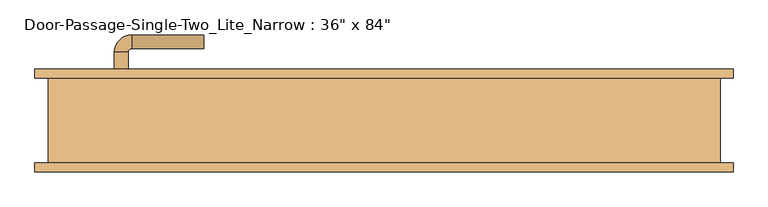
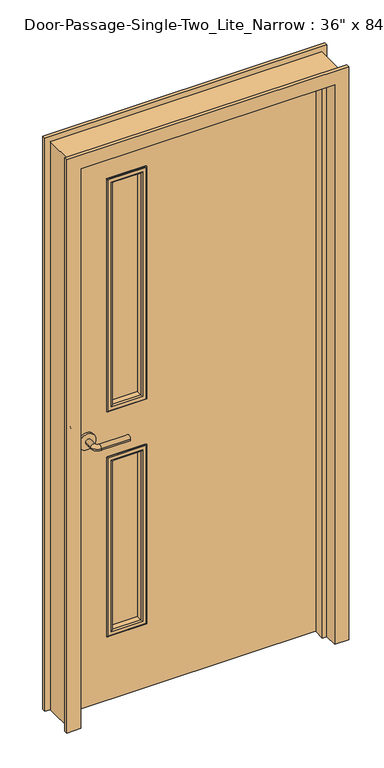
"""IFC4 building model written with IfcOpenShell, lengths in millimetres: door geometry."""

import ifcopenshell
import ifcopenshell.guid

model = None  # the IFC model being written
_history = None  # IfcOwnerHistory: only IFC2X3 demands one
_inside = {}  # id of a spatial element -> (the spatial element, [elements in it])
_under = {}  # id of a project, library or spatial element -> (it, [spatial elements below it])
_declared = {}  # id of a project -> (the project, [libraries it declares])
_typed = {}  # id of a type object -> (the type object, [elements of that type])
_made_of = {}  # id of a material, layer set ... -> (it, [elements and type objects made of it])


def new_model(schema):
    """Start an empty IFC model of exactly this schema.

    Asked for "IFC4X3", IfcOpenShell would pick the latest addendum, in which some entities
    have other attributes; the version numbers below select the first issue.
    IFC2X3 requires an IfcOwnerHistory on every rooted entity: one is made here for all.
    """
    global model, _history
    if schema == "IFC4X3":
        model = ifcopenshell.file(schema_version=(4, 3, 0, 0))
    else:
        model = ifcopenshell.file(schema=schema)
    _inside.clear()
    _under.clear()
    _declared.clear()
    _typed.clear()
    _made_of.clear()
    _history = None
    if model.schema == "IFC2X3":
        org = make("IfcOrganization", Name="unknown")
        user = make(
            "IfcPersonAndOrganization",
            ThePerson=make("IfcPerson", FamilyName="unknown"),
            TheOrganization=org,
        )
        app = make(
            "IfcApplication",
            ApplicationDeveloper=org,
            Version="unknown",
            ApplicationFullName="unknown",
            ApplicationIdentifier="unknown",
        )
        _history = make(
            "IfcOwnerHistory",
            OwningUser=user,
            OwningApplication=app,
            ChangeAction="ADDED",
            CreationDate=0,
        )
    return model


def make(cls, **values):
    """One entity of the class cls with the attributes given. An attribute that is None is left unset."""
    return model.create_entity(
        cls, **{name: value for name, value in values.items() if value is not None}
    )


def rooted(cls, **values):
    """An entity with a GlobalId (a new one), such as an element, a storey or a relation."""
    return make(cls, GlobalId=ifcopenshell.guid.new(), OwnerHistory=_history, **values)


def si_unit(unit_type, name, prefix=None):
    """IfcSIUnit, for example si_unit("LENGTHUNIT", "METRE", prefix="MILLI")."""
    return make("IfcSIUnit", UnitType=unit_type, Prefix=prefix, Name=name)


def assignment(units):
    """IfcUnitAssignment: the units of a project."""
    return None if units is None else make("IfcUnitAssignment", Units=units)


def point(xyz):
    """IfcCartesianPoint."""
    return None if xyz is None else make("IfcCartesianPoint", Coordinates=xyz)


def direction(xyz):
    """IfcDirection."""
    return None if xyz is None else make("IfcDirection", DirectionRatios=xyz)


def frame(location, z_axis=None, x_axis=None):
    """IfcAxis2Placement3D, a coordinate frame: its origin and axes. An axis left out is left unset."""
    return make(
        "IfcAxis2Placement3D",
        Location=point(location),
        Axis=direction(z_axis),
        RefDirection=direction(x_axis),
    )


def frame_2d(location, x_axis=None):
    """IfcAxis2Placement2D, a coordinate frame in the plane: its origin and x axis."""
    return make(
        "IfcAxis2Placement2D", Location=point(location), RefDirection=direction(x_axis)
    )


def origin():
    """The frame at (0, 0, 0) with its axes left unset."""
    return frame((0.0, 0.0, 0.0))


def place(relative_to, where):
    """IfcLocalPlacement: puts the frame where relative to a parent placement (None: the world)."""
    return make(
        "IfcLocalPlacement", PlacementRelTo=relative_to, RelativePlacement=where
    )


def context(
    kind, dimensions, precision=None, world=None, true_north=None, identifier=None
):
    """IfcGeometricRepresentationContext, for example the 3D "Model" context."""
    return make(
        "IfcGeometricRepresentationContext",
        ContextIdentifier=identifier,
        ContextType=kind,
        CoordinateSpaceDimension=dimensions,
        Precision=precision,
        WorldCoordinateSystem=world,
        TrueNorth=true_north,
    )


def project(units=None, contexts=None):
    """IfcProject with its units and contexts."""
    return rooted(
        "IfcProject",
        Name="project",
        RepresentationContexts=contexts,
        UnitsInContext=assignment(units),
    )


def spatial(cls, under=None, at=None, **own):
    """A site, building, storey or space (cls), placed at a placement, below another one or the project."""
    s = rooted(cls, ObjectPlacement=at, **own)
    if under is not None:
        _under.setdefault(under.id(), (under, []))[1].append(s)
    return s


def polyline(points):
    """IfcPolyline through the points."""
    return make("IfcPolyline", Points=[point(p) for p in points])


def circle_curve(where, radius):
    """IfcCircle in the frame where."""
    return make("IfcCircle", Position=where, Radius=radius)


def ellipse_curve(where, semi_axis1, semi_axis2):
    """IfcEllipse in the frame where."""
    return make(
        "IfcEllipse", Position=where, SemiAxis1=semi_axis1, SemiAxis2=semi_axis2
    )


def trimmed(basis, trim1, trim2, sense, master):
    """IfcTrimmedCurve: the piece of a basis curve between two trims."""
    return make(
        "IfcTrimmedCurve",
        BasisCurve=basis,
        Trim1=trim1,
        Trim2=trim2,
        SenseAgreement=sense,
        MasterRepresentation=master,
    )


def segment(curve, same_sense, transition):
    """IfcCompositeCurveSegment."""
    return make(
        "IfcCompositeCurveSegment",
        Transition=transition,
        SameSense=same_sense,
        ParentCurve=curve,
    )


def composite_curve(segments, self_intersect=None):
    """IfcCompositeCurve: segments joined end to end."""
    return make("IfcCompositeCurve", Segments=segments, SelfIntersect=self_intersect)


def outline(outer, holes=None, kind="AREA"):
    """IfcArbitraryClosedProfileDef: a profile drawn as a closed curve; with holes, ...WithVoids."""
    if holes is None:
        return make("IfcArbitraryClosedProfileDef", ProfileType=kind, OuterCurve=outer)
    return make(
        "IfcArbitraryProfileDefWithVoids",
        ProfileType=kind,
        OuterCurve=outer,
        InnerCurves=holes,
    )


def extrude(swept, where, along, depth):
    """IfcExtrudedAreaSolid: the profile swept, set in the frame where, extruded along a direction by depth."""
    return make(
        "IfcExtrudedAreaSolid",
        SweptArea=swept,
        Position=where,
        ExtrudedDirection=direction(along),
        Depth=depth,
    )


def faces_of(points, faces, orient=None, outer=None):
    """IfcFace entities. A face is a list of loops; a loop is a list of indices into points, from 0.

    orient and outer hold one flag for each loop. By default every Orientation is true, the
    first loop of a face is its IfcFaceOuterBound and the others are IfcFaceBound.
    """
    made = []
    for i, loops in enumerate(faces):
        bounds = []
        for j, loop in enumerate(loops):
            is_outer = j == 0 if outer is None else outer[i][j]
            bounds.append(
                make(
                    "IfcFaceOuterBound" if is_outer else "IfcFaceBound",
                    Bound=make("IfcPolyLoop", Polygon=[points[k] for k in loop]),
                    Orientation=True if orient is None else orient[i][j],
                )
            )
        made.append(make("IfcFace", Bounds=bounds))
    return made


def faceted_brep(points, faces, orient=None, outer=None, voids=None):
    """IfcFacetedBrep: a solid bounded by flat faces; with voids (closed shells), ...WithVoids."""
    shared = [point(p) for p in points]
    hull = make("IfcClosedShell", CfsFaces=faces_of(shared, faces, orient, outer))
    if voids is None:
        return make("IfcFacetedBrep", Outer=hull)
    return make(
        "IfcFacetedBrepWithVoids",
        Outer=hull,
        Voids=[
            make(cls, CfsFaces=faces_of(shared, fs, o, b)) for cls, fs, o, b in voids
        ],
    )


def shape(context_of_items, identifier, shape_type, items):
    """IfcShapeRepresentation: the items that make up one representation, for example the "Body"."""
    return make(
        "IfcShapeRepresentation",
        ContextOfItems=context_of_items,
        RepresentationIdentifier=identifier,
        RepresentationType=shape_type,
        Items=items,
    )


def source(mapping_origin, context_of_items, identifier, shape_type, items):
    """IfcRepresentationMap: a shape defined once, which mapped items show again and again."""
    return make(
        "IfcRepresentationMap",
        MappingOrigin=mapping_origin,
        MappedRepresentation=shape(context_of_items, identifier, shape_type, items),
    )


def transform(
    local_origin,
    x_axis=None,
    y_axis=None,
    z_axis=None,
    scale=None,
    scale2=None,
    scale3=None,
    uniform=True,
):
    """IfcCartesianTransformationOperator3D, or its non-uniform kind. x_axis, y_axis, z_axis: its Axis1, 2, 3."""
    if uniform:
        return make(
            "IfcCartesianTransformationOperator3D",
            Axis1=direction(x_axis),
            Axis2=direction(y_axis),
            LocalOrigin=point(local_origin),
            Scale=scale,
            Axis3=direction(z_axis),
        )
    return make(
        "IfcCartesianTransformationOperator3DnonUniform",
        Axis1=direction(x_axis),
        Axis2=direction(y_axis),
        LocalOrigin=point(local_origin),
        Scale=scale,
        Axis3=direction(z_axis),
        Scale2=scale2,
        Scale3=scale3,
    )


def mapped(mapping_source, mapping_target):
    """IfcMappedItem: shows the shape of a source again, moved by a transform."""
    return make(
        "IfcMappedItem", MappingSource=mapping_source, MappingTarget=mapping_target
    )


def made_of(thing, what):
    """Note that an element or type object is made of a material, layer set ...; save() writes the relation."""
    if what is not None:
        _made_of.setdefault(what.id(), (what, []))[1].append(thing)
    return thing


def element(
    cls,
    number,
    at=None,
    inside=None,
    cuts=None,
    type_object=None,
    material=None,
    context=None,
    identifier="Body",
    shape_type=None,
    held_by="IfcProductDefinitionShape",
    body=None,
    shapes=None,
    **own,
):
    """One element of the class cls, such as IfcWall. Its Tag is "e" and its number.

    at: its placement. inside: the storey or other place that contains it. cuts: it is an
    opening in that element (IfcRelVoidsElement). A single representation is given by context,
    identifier, shape_type and body (its items); several are given by shapes. held_by: the class
    of the entity that holds the representations. save() writes the other relations.
    """
    e = rooted(cls, Tag="e%d" % number, ObjectPlacement=at, **own)
    if body is not None:
        shapes = [shape(context, identifier, shape_type, body)]
    if shapes is not None:
        e.Representation = make(held_by, Representations=shapes)
    if inside is not None:
        _inside.setdefault(inside.id(), (inside, []))[1].append(e)
    if cuts is not None:
        rooted(
            "IfcRelVoidsElement", RelatingBuildingElement=cuts, RelatedOpeningElement=e
        )
    if type_object is not None:
        _typed.setdefault(type_object.id(), (type_object, []))[1].append(e)
    return made_of(e, material)


def aggregate(whole, parts):
    """IfcRelAggregates: a whole, such as a stair, and the parts it consists of."""
    return rooted("IfcRelAggregates", RelatingObject=whole, RelatedObjects=parts)


def save(model, path):
    """Write the relations noted so far, then the file.

    IfcRelAggregates (storeys below a building ...), IfcRelContainedInSpatialStructure (elements
    in a storey), IfcRelDefinesByType, IfcRelAssociatesMaterial and IfcRelDeclares: one each for
    every whole, place, type object, material and project.
    """
    for whole, parts in _under.values():
        aggregate(whole, parts)
    for where, things in _inside.values():
        rooted(
            "IfcRelContainedInSpatialStructure",
            RelatedElements=things,
            RelatingStructure=where,
        )
    for kind, things in _typed.values():
        rooted("IfcRelDefinesByType", RelatedObjects=things, RelatingType=kind)
    for what, things in _made_of.values():
        rooted("IfcRelAssociatesMaterial", RelatedObjects=things, RelatingMaterial=what)
    for by, libraries in _declared.values():
        rooted("IfcRelDeclares", RelatingContext=by, RelatedDefinitions=libraries)
    model.write(path)


def plane_surface(at):
    """IfcPlane: the flat surface through the origin of the frame at, square to its z axis."""
    return make("IfcPlane", Position=at)


def cylinder_surface(at, radius):
    """IfcCylindricalSurface: all points at the distance radius from the z axis of the frame at."""
    return make("IfcCylindricalSurface", Position=at, Radius=radius)


def revolved_surface(curve, axis_point, axis_direction):
    """IfcSurfaceOfRevolution: the curve turned about the line through axis_point along axis_direction."""
    return make(
        "IfcSurfaceOfRevolution",
        SweptCurve=make("IfcArbitraryOpenProfileDef", ProfileType="CURVE", Curve=curve),
        AxisPosition=make("IfcAxis1Placement", Location=point(axis_point), Axis=direction(axis_direction)),
    )


def advanced_brep(points, edges, surfaces, faces):
    """IfcAdvancedBrep: a solid bounded by faces that lie on surfaces and meet in shared edges.

    An edge is (start, end): straight between two places in points (the first is 0);
    or (start, end, curve); or (start, end, curve, False) where it runs against its curve.
    A face is (place in surfaces, loops), or (place, loops, False) where it looks against
    its surface's normal. A loop lists edges by number (the first is 1), with a minus sign
    where the edge is run from its end to its start. The first loop is the outer one.
    """
    corners = [point(p) for p in points]
    vertices = [make("IfcVertexPoint", VertexGeometry=c) for c in corners]
    made = []
    for start, end, *more in edges:
        made.append(
            make(
                "IfcEdgeCurve",
                EdgeStart=vertices[start],
                EdgeEnd=vertices[end],
                EdgeGeometry=more[0] if more else make("IfcPolyline", Points=[corners[start], corners[end]]),
                SameSense=more[1] if len(more) > 1 else True,
            )
        )
    hull = []
    for where, loops, *sense in faces:
        bounds = []
        for j, loop in enumerate(loops):
            ring = [make("IfcOrientedEdge", EdgeElement=made[abs(k) - 1], Orientation=k > 0) for k in loop]
            bounds.append(
                make(
                    "IfcFaceOuterBound" if j == 0 else "IfcFaceBound",
                    Bound=make("IfcEdgeLoop", EdgeList=ring),
                    Orientation=True,
                )
            )
        hull.append(make("IfcAdvancedFace", Bounds=bounds, FaceSurface=surfaces[where], SameSense=sense[0] if sense else True))
    return make("IfcAdvancedBrep", Outer=make("IfcClosedShell", CfsFaces=hull))


def door_dba893c0(model_context):
    return source(origin(), model_context, "Body", "SolidModel", [
        advanced_brep(
        [(-392.190625, 15.8125, 1016.0), (-372.190625, 15.8125, 1016.0), (-372.190625, -14.1875, 1016.0), (-392.190625, -14.1875, 1016.0), (-367.190625, -19.1875, 1016.0), (-367.190625, -39.1875, 1016.0), (-262.190625, -39.1875, 1016.0), (-262.190625, -19.1875, 1016.0)],
        [
            (0, 1, circle_curve(frame((-382.190625, 15.8125, 1016.0), z_axis=(0.0, 1.0, 0.0), x_axis=(1.0, 0.0, 0.0)), 10.0)),
            (1, 0, circle_curve(frame((-382.190625, 15.8125, 1016.0), z_axis=(0.0, 1.0, 0.0), x_axis=(1.0, 0.0, 0.0)), 10.0)),
            (1, 2),
            (2, 3, circle_curve(frame((-382.190625, -14.1875, 1016.0), z_axis=(0.0, 1.0, 0.0), x_axis=(1.0, 0.0, 0.0)), 10.0)),
            (3, 0),
            (3, 2, circle_curve(frame((-382.190625, -14.1875, 1016.0), z_axis=(0.0, 1.0, 0.0), x_axis=(1.0, 0.0, 0.0)), 10.0)),
            (4, 5, circle_curve(frame((-367.190625, -29.1875, 1016.0), z_axis=(-1.0, 0.0, 0.0), x_axis=(0.0, 1.0, 0.0)), 10.0)),
            (5, 3, circle_curve(frame((-367.190625, -14.1875, 1016.0), z_axis=(0.0, 0.0, -1.0), x_axis=(-1.0, 0.0, 0.0)), 25.0)),
            (2, 4, circle_curve(frame((-367.190625, -14.1875, 1016.0), z_axis=(0.0, 0.0, 1.0), x_axis=(-1.0, 0.0, 0.0)), 5.0)),
            (5, 4, circle_curve(frame((-367.190625, -29.1875, 1016.0), z_axis=(-1.0, 0.0, 0.0), x_axis=(0.0, 1.0, 0.0)), 10.0)),
            (6, 7, circle_curve(frame((-262.190625, -29.1875, 1016.0), z_axis=(1.0, 0.0, 0.0), x_axis=(0.0, 1.0, 0.0)), 10.0)),
            (7, 6, circle_curve(frame((-262.190625, -29.1875, 1016.0), z_axis=(1.0, 0.0, 0.0), x_axis=(0.0, 1.0, 0.0)), 10.0)),
            (4, 7),
            (6, 5),
        ],
        [
            plane_surface(frame((-382.190625, 15.8125, 1016.0), z_axis=(0.0, 1.0, 0.0), x_axis=(0.0, 0.0, 1.0))),
            cylinder_surface(frame((-382.190625, 15.8125, 1016.0), z_axis=(0.0, 1.0, 0.0), x_axis=(1.0, 0.0, 0.0)), 10.0),
            revolved_surface(trimmed(ellipse_curve(frame((-382.190625, -14.1875, 1016.0), z_axis=(0.0, -1.0, 0.0), x_axis=(1.0, 0.0, 0.0)), 10.0, 10.0), [point((-392.190625, -14.1875, 1016.0))], [point((-372.190625, -14.1875, 1016.0))], True, "CARTESIAN"), (-367.190625, -14.1875, 1016.0), (0.0, 0.0, -1.0)),
            revolved_surface(trimmed(ellipse_curve(frame((-382.190625, -14.1875, 1016.0), z_axis=(0.0, -1.0, 0.0), x_axis=(1.0, 0.0, 0.0)), 10.0, 10.0), [point((-372.190625, -14.1875, 1016.0))], [point((-392.190625, -14.1875, 1016.0))], True, "CARTESIAN"), (-367.190625, -14.1875, 1016.0), (0.0, 0.0, -1.0)),
            plane_surface(frame((-262.190625, -29.1875, 1016.0), z_axis=(1.0, 0.0, 0.0), x_axis=(0.0, 0.0, 1.0))),
            cylinder_surface(frame((-367.190625, -29.1875, 1016.0), z_axis=(-1.0, 0.0, 0.0), x_axis=(0.0, 1.0, 0.0)), 10.0),
        ],
        [
            (0, [[1, 2]]),
            (1, [[3, 4, 5, -2]]),
            (1, [[-5, 6, -3, -1]]),
            (2, [[7, 8, -4, 9]]),
            (3, [[10, -9, -6, -8]]),
            (4, [[11, 12]]),
            (5, [[13, -11, 14, -7]]),
            (5, [[-14, -12, -13, -10]]),
        ],
    ),
        extrude(outline(composite_curve([segment(trimmed(circle_curve(frame_2d((1016.0, -384.690625)), 30.0), [point((1016.0, -414.690625))], [point((1016.0, -354.690625))], False, "CARTESIAN"), True, "CONTINUOUS"), segment(trimmed(circle_curve(frame_2d((1016.0, -384.690625)), 30.0), [point((1016.0, -354.690625))], [point((1016.0, -414.690625))], False, "CARTESIAN"), True, "CONTINUOUS")], self_intersect=False)), frame((0.0, 15.8125, 0.0), z_axis=(0.0, 1.0, 0.0), x_axis=(0.0, 0.0, 1.0)), (0.0, 0.0, 1.0), 8.0),
        advanced_brep(
        [(-392.190625, 76.2625, 1016.0), (-372.190625, 76.2625, 1016.0), (-392.190625, 106.2625, 1016.0), (-372.190625, 106.2625, 1016.0), (-367.190625, 111.2625, 1016.0), (-367.190625, 131.2625, 1016.0), (-262.190625, 131.2625, 1016.0), (-262.190625, 111.2625, 1016.0)],
        [
            (0, 1, circle_curve(frame((-382.190625, 76.2625, 1016.0), z_axis=(0.0, -1.0, 0.0), x_axis=(1.0, 0.0, 0.0)), 10.0)),
            (1, 0, circle_curve(frame((-382.190625, 76.2625, 1016.0), z_axis=(0.0, -1.0, 0.0), x_axis=(1.0, 0.0, 0.0)), 10.0)),
            (0, 2),
            (2, 3, circle_curve(frame((-382.190625, 106.2625, 1016.0), z_axis=(0.0, -1.0, 0.0), x_axis=(1.0, 0.0, 0.0)), 10.0)),
            (3, 1),
            (3, 2, circle_curve(frame((-382.190625, 106.2625, 1016.0), z_axis=(0.0, -1.0, 0.0), x_axis=(1.0, 0.0, 0.0)), 10.0)),
            (4, 3, circle_curve(frame((-367.190625, 106.2625, 1016.0), z_axis=(0.0, 0.0, 1.0), x_axis=(-1.0, 0.0, 0.0)), 5.0)),
            (2, 5, circle_curve(frame((-367.190625, 106.2625, 1016.0), z_axis=(0.0, 0.0, -1.0), x_axis=(-1.0, 0.0, 0.0)), 25.0)),
            (5, 4, circle_curve(frame((-367.190625, 121.2625, 1016.0), z_axis=(-1.0, 0.0, 0.0), x_axis=(0.0, -1.0, 0.0)), 10.0)),
            (4, 5, circle_curve(frame((-367.190625, 121.2625, 1016.0), z_axis=(-1.0, 0.0, 0.0), x_axis=(0.0, -1.0, 0.0)), 10.0)),
            (6, 7, circle_curve(frame((-262.190625, 121.2625, 1016.0), z_axis=(1.0, 0.0, 0.0), x_axis=(0.0, -1.0, 0.0)), 10.0)),
            (7, 6, circle_curve(frame((-262.190625, 121.2625, 1016.0), z_axis=(1.0, 0.0, 0.0), x_axis=(0.0, -1.0, 0.0)), 10.0)),
            (5, 6),
            (7, 4),
        ],
        [
            plane_surface(frame((-382.190625, 76.2625, 1016.0), z_axis=(0.0, -1.0, 0.0), x_axis=(0.0, 0.0, 1.0))),
            cylinder_surface(frame((-382.190625, 76.2625, 1016.0), z_axis=(0.0, -1.0, 0.0), x_axis=(1.0, 0.0, 0.0)), 10.0),
            revolved_surface(trimmed(ellipse_curve(frame((-382.190625, 106.2625, 1016.0), z_axis=(0.0, -1.0, 0.0), x_axis=(1.0, 0.0, 0.0)), 10.0, 10.0), [point((-392.190625, 106.2625, 1016.0))], [point((-372.190625, 106.2625, 1016.0))], True, "CARTESIAN"), (-367.190625, 106.2625, 1016.0), (0.0, 0.0, -1.0)),
            revolved_surface(trimmed(ellipse_curve(frame((-382.190625, 106.2625, 1016.0), z_axis=(0.0, -1.0, 0.0), x_axis=(1.0, 0.0, 0.0)), 10.0, 10.0), [point((-372.190625, 106.2625, 1016.0))], [point((-392.190625, 106.2625, 1016.0))], True, "CARTESIAN"), (-367.190625, 106.2625, 1016.0), (0.0, 0.0, -1.0)),
            plane_surface(frame((-262.190625, 121.2625, 1016.0), z_axis=(1.0, 0.0, 0.0), x_axis=(0.0, 0.0, 1.0))),
            cylinder_surface(frame((-367.190625, 121.2625, 1016.0), z_axis=(-1.0, 0.0, 0.0), x_axis=(0.0, -1.0, 0.0)), 10.0),
        ],
        [
            (0, [[1, 2]]),
            (1, [[-1, 3, 4, 5]]),
            (1, [[-2, -5, 6, -3]]),
            (2, [[7, -4, 8, 9]]),
            (3, [[-8, -6, -7, 10]]),
            (4, [[11, 12]]),
            (5, [[-9, 13, -12, 14]]),
            (5, [[-10, -14, -11, -13]]),
        ],
    ),
        extrude(outline(composite_curve([segment(trimmed(circle_curve(frame_2d((1016.0, -384.690625)), 30.0), [point((1016.0, -414.690625))], [point((1016.0, -354.690625))], False, "CARTESIAN"), True, "CONTINUOUS"), segment(trimmed(circle_curve(frame_2d((1016.0, -384.690625)), 30.0), [point((1016.0, -354.690625))], [point((1016.0, -414.690625))], False, "CARTESIAN"), True, "CONTINUOUS")], self_intersect=False)), frame((0.0, 68.2625, 0.0), z_axis=(0.0, 1.0, 0.0), x_axis=(0.0, 0.0, 1.0)), (0.0, 0.0, 1.0), 8.0),
        faceted_brep([(457.2, 80.9625, 0.0), (508.0, 80.9625, 0.0), (508.0, 68.2625, 0.0), (488.95, 68.2625, 0.0), (488.95, -55.5625, 0.0), (508.0, -55.5625, 0.0), (508.0, -68.2625, 0.0), (457.2, -68.2625, 0.0), (457.2, -19.05, 0.0), (441.325, -19.05, 0.0), (441.325, 19.05, 0.0), (457.2, 19.05, 0.0), (457.2, 80.9625, 2133.6), (-457.2, 80.9625, 2133.6), (-457.2, 80.9625, 0.0), (-508.0, 80.9625, 0.0), (-508.0, 80.9625, 2184.4), (508.0, 80.9625, 2184.4), (508.0, 68.2625, 2184.4), (-508.0, 68.2625, 2184.4), (-508.0, 68.2625, 0.0), (-488.95, 68.2625, 0.0), (-488.95, 68.2625, 2165.35), (488.95, 68.2625, 2165.35), (488.95, -55.5625, 2165.35), (-488.95, -55.5625, 2165.35), (-488.95, -55.5625, 0.0), (-508.0, -55.5625, 0.0), (-508.0, -55.5625, 2184.4), (508.0, -55.5625, 2184.4), (508.0, -68.2625, 2184.4), (-508.0, -68.2625, 2184.4), (-508.0, -68.2625, 0.0), (-457.2, -68.2625, 0.0), (-457.2, -68.2625, 2133.6), (457.2, -68.2625, 2133.6), (457.2, -19.05, 2133.6), (-457.2, -19.05, 2133.6), (-457.2, -19.05, 0.0), (-441.325, -19.05, 0.0), (-441.325, -19.05, 2117.725), (441.325, -19.05, 2117.725), (441.325, 19.05, 2117.725), (-441.325, 19.05, 2117.725), (-441.325, 19.05, 0.0), (-457.2, 19.05, 0.0), (-457.2, 19.05, 2133.6), (457.2, 19.05, 2133.6)], [[[0, 1, 2, 3, 4, 5, 6, 7, 8, 9, 10, 11]], [[1, 0, 12, 13, 14, 15, 16, 17]], [[2, 1, 17, 18]], [[3, 2, 18, 19, 20, 21, 22, 23]], [[4, 3, 23, 24]], [[5, 4, 24, 25, 26, 27, 28, 29]], [[6, 5, 29, 30]], [[7, 6, 30, 31, 32, 33, 34, 35]], [[8, 7, 35, 36]], [[9, 8, 36, 37, 38, 39, 40, 41]], [[10, 9, 41, 42]], [[11, 10, 42, 43, 44, 45, 46, 47]], [[0, 11, 47, 12]], [[18, 17, 16, 19]], [[24, 23, 22, 25]], [[30, 29, 28, 31]], [[36, 35, 34, 37]], [[42, 41, 40, 43]], [[12, 47, 46, 13]], [[14, 45, 44, 39, 38, 33, 32, 27, 26, 21, 20, 15]], [[19, 16, 15, 20]], [[25, 22, 21, 26]], [[31, 28, 27, 32]], [[37, 34, 33, 38]], [[43, 40, 39, 44]], [[13, 46, 45, 14]]]),
        extrude(outline(polyline([(2133.6, -457.2), (0.0, -457.2), (0.0, 457.2), (2133.6, 457.2), (2133.6, -457.2)]), holes=[polyline([(1981.2, -304.8), (1981.2, -177.8), (1111.25, -177.8), (1111.25, -304.8), (1981.2, -304.8)]), polyline([(920.75, -304.8), (920.75, -177.8), (254.0, -177.8), (254.0, -304.8), (920.75, -304.8)])]), frame((0.0, 23.8125, 0.0), z_axis=(0.0, 1.0, 0.0), x_axis=(0.0, 0.0, 1.0)), (0.0, 0.0, 1.0), 44.45),
        extrude(outline(polyline([(-177.8, 42.8625), (-304.8, 42.8625), (-304.8, 49.2125), (-177.8, 49.2125), (-177.8, 42.8625)])), frame((0.0, 0.0, 1111.25), z_axis=(0.0, 0.0, 1.0), x_axis=(1.0, 0.0, 0.0)), (0.0, 0.0, 1.0), 869.95),
        extrude(outline(polyline([(-177.8, 42.8625), (-304.8, 42.8625), (-304.8, 49.2125), (-177.8, 49.2125), (-177.8, 42.8625)])), frame((0.0, 0.0, 254.0), z_axis=(0.0, 0.0, 1.0), x_axis=(1.0, 0.0, 0.0)), (0.0, 0.0, 1.0), 666.75),
        advanced_brep(
        [(-177.8, 42.8625, 920.75), (-177.8, 23.8125, 920.75), (-177.8, 23.8125, 254.0), (-177.8, 42.8625, 254.0), (-189.8, 22.8125, 908.75), (-189.8, 42.8625, 908.75), (-189.8, 42.8625, 266.0), (-189.8, 22.8125, 266.0), (-184.8, 17.8125, 913.75), (-184.8, 17.8125, 261.0), (-169.8, 19.8125, 928.75), (-171.8, 17.8125, 926.75), (-171.8, 17.8125, 248.0), (-169.8, 19.8125, 246.0), (-169.8, 23.8125, 928.75), (-169.8, 23.8125, 246.0), (-304.8, 23.8125, 254.0), (-304.8, 42.8625, 254.0), (-292.8, 42.8625, 266.0), (-292.8, 22.8125, 266.0), (-297.8, 17.8125, 261.0), (-310.8, 17.8125, 248.0), (-312.8, 19.8125, 246.0), (-312.8, 23.8125, 246.0), (-304.8, 23.8125, 920.75), (-304.8, 42.8625, 920.75), (-292.8, 42.8625, 908.75), (-292.8, 22.8125, 908.75), (-297.8, 17.8125, 913.75), (-310.8, 17.8125, 926.75), (-312.8, 19.8125, 928.75), (-312.8, 23.8125, 928.75)],
        [
            (0, 1),
            (1, 2),
            (2, 3),
            (3, 0),
            (4, 5),
            (5, 6),
            (6, 7),
            (7, 4),
            (8, 4, ellipse_curve(frame((-184.8, 22.8125, 913.75), z_axis=(0.7071067811865475, 0.0, -0.7071067811865475), x_axis=(0.7071067811865474, 0.0, 0.7071067811865476)), 7.0710678, 5.0)),
            (7, 9, ellipse_curve(frame((-184.8, 22.8125, 261.0), z_axis=(0.7071067811865475, 0.0, 0.7071067811865475), x_axis=(-0.7071067811865474, 0.0, 0.7071067811865476)), 7.0710678, 5.0)),
            (9, 8),
            (10, 11, ellipse_curve(frame((-171.8, 19.8125, 926.75), z_axis=(0.7071067811865475, 0.0, -0.7071067811865475), x_axis=(0.7071067811865474, 0.0, 0.7071067811865476)), 2.8284271, 2.0)),
            (11, 12),
            (12, 13, ellipse_curve(frame((-171.8, 19.8125, 248.0), z_axis=(0.7071067811865475, 0.0, 0.7071067811865475), x_axis=(-0.7071067811865474, 0.0, 0.7071067811865476)), 2.8284271, 2.0)),
            (13, 10),
            (14, 10),
            (13, 15),
            (15, 14),
            (2, 16),
            (16, 17),
            (17, 3),
            (6, 18),
            (18, 19),
            (19, 7),
            (19, 20, ellipse_curve(frame((-297.8, 22.8125, 261.0), z_axis=(0.7071067811865475, 0.0, -0.7071067811865475), x_axis=(0.7071067811865476, 0.0, 0.7071067811865474)), 7.0710678, 5.0)),
            (20, 9),
            (12, 21),
            (21, 22, ellipse_curve(frame((-310.8, 19.8125, 248.0), z_axis=(0.7071067811865475, 0.0, -0.7071067811865475), x_axis=(0.7071067811865476, 0.0, 0.7071067811865474)), 2.8284271, 2.0)),
            (22, 13),
            (22, 23),
            (23, 15),
            (16, 24),
            (24, 25),
            (25, 17),
            (18, 26),
            (26, 27),
            (27, 19),
            (27, 28, ellipse_curve(frame((-297.8, 22.8125, 913.75), z_axis=(-0.7071067811865475, 0.0, -0.7071067811865475), x_axis=(0.7071067811865474, 0.0, -0.7071067811865476)), 7.0710678, 5.0)),
            (28, 20),
            (21, 29),
            (29, 30, ellipse_curve(frame((-310.8, 19.8125, 926.75), z_axis=(-0.7071067811865475, 0.0, -0.7071067811865475), x_axis=(0.7071067811865474, 0.0, -0.7071067811865476)), 2.8284271, 2.0)),
            (30, 22),
            (30, 31),
            (31, 23),
            (31, 14),
            (1, 24),
            (0, 25),
            (5, 26),
            (4, 27),
            (8, 28),
            (11, 29),
            (10, 30),
        ],
        [
            plane_surface(frame((-177.8, 23.8125, 920.75), z_axis=(1.0, 0.0, 0.0), x_axis=(0.0, 0.0, -1.0))),
            plane_surface(frame((-189.8, 42.8625, 908.75), z_axis=(-1.0, 0.0, 0.0), x_axis=(0.0, 0.0, -1.0))),
            cylinder_surface(frame((-184.8, 22.8125, 920.75), z_axis=(0.0, 0.0, 1.0), x_axis=(1.0, 0.0, 0.0)), 5.0),
            cylinder_surface(frame((-171.8, 19.8125, 920.75), z_axis=(0.0, 0.0, 1.0), x_axis=(1.0, 0.0, 0.0)), 2.0),
            plane_surface(frame((-169.8, 19.8125, 928.75), z_axis=(1.0, 0.0, 0.0), x_axis=(0.0, 0.0, -1.0))),
            plane_surface(frame((-177.8, 23.8125, 254.0), z_axis=(0.0, 0.0, -1.0), x_axis=(-1.0, 0.0, 0.0))),
            plane_surface(frame((-189.8, 42.8625, 266.0), z_axis=(0.0, 0.0, 1.0), x_axis=(-1.0, 0.0, 0.0))),
            cylinder_surface(frame((-177.8, 22.8125, 261.0), z_axis=(1.0, 0.0, 0.0), x_axis=(0.0, 0.0, -1.0)), 5.0),
            cylinder_surface(frame((-177.8, 19.8125, 248.0), z_axis=(1.0, 0.0, 0.0), x_axis=(0.0, 0.0, -1.0)), 2.0),
            plane_surface(frame((-169.8, 19.8125, 246.0), z_axis=(0.0, 0.0, -1.0), x_axis=(-1.0, 0.0, 0.0))),
            plane_surface(frame((-304.8, 23.8125, 254.0), z_axis=(-1.0, 0.0, 0.0), x_axis=(0.0, 0.0, 1.0))),
            plane_surface(frame((-292.8, 42.8625, 266.0), z_axis=(1.0, 0.0, 0.0), x_axis=(0.0, 0.0, 1.0))),
            cylinder_surface(frame((-297.8, 22.8125, 254.0), z_axis=(0.0, 0.0, -1.0), x_axis=(-1.0, 0.0, 0.0)), 5.0),
            cylinder_surface(frame((-310.8, 19.8125, 254.0), z_axis=(0.0, 0.0, -1.0), x_axis=(-1.0, 0.0, 0.0)), 2.0),
            plane_surface(frame((-312.8, 19.8125, 246.0), z_axis=(-1.0, 0.0, 0.0), x_axis=(0.0, 0.0, 1.0))),
            plane_surface(frame((-312.8, 23.8125, 928.75), z_axis=(0.0, 1.0, 0.0), x_axis=(1.0, 0.0, 0.0))),
            plane_surface(frame((-304.8, 23.8125, 920.75), z_axis=(0.0, 0.0, 1.0), x_axis=(1.0, 0.0, 0.0))),
            plane_surface(frame((-304.8, 42.8625, 920.75), z_axis=(0.0, 1.0, 0.0), x_axis=(1.0, 0.0, 0.0))),
            plane_surface(frame((-292.8, 42.8625, 908.75), z_axis=(0.0, 0.0, -1.0), x_axis=(1.0, 0.0, 0.0))),
            cylinder_surface(frame((-304.8, 22.8125, 913.75), z_axis=(-1.0, 0.0, 0.0), x_axis=(0.0, 0.0, 1.0)), 5.0),
            plane_surface(frame((-297.8, 17.8125, 913.75), z_axis=(0.0, -1.0, 0.0), x_axis=(1.0, 0.0, 0.0))),
            cylinder_surface(frame((-304.8, 19.8125, 926.75), z_axis=(-1.0, 0.0, 0.0), x_axis=(0.0, 0.0, 1.0)), 2.0),
            plane_surface(frame((-312.8, 19.8125, 928.75), z_axis=(0.0, 0.0, 1.0), x_axis=(1.0, 0.0, 0.0))),
        ],
        [
            (0, [[1, 2, 3, 4]]),
            (1, [[5, 6, 7, 8]]),
            (2, [[9, -8, 10, 11]]),
            (3, [[12, 13, 14, 15]]),
            (4, [[16, -15, 17, 18]]),
            (5, [[-3, 19, 20, 21]]),
            (6, [[-7, 22, 23, 24]]),
            (7, [[-10, -24, 25, 26]]),
            (8, [[-14, 27, 28, 29]]),
            (9, [[-17, -29, 30, 31]]),
            (10, [[-20, 32, 33, 34]]),
            (11, [[-23, 35, 36, 37]]),
            (12, [[-25, -37, 38, 39]]),
            (13, [[-28, 40, 41, 42]]),
            (14, [[-30, -42, 43, 44]]),
            (15, [[-31, -44, 45, -18], [46, -32, -19, -2]]),
            (16, [[-33, -46, -1, 47]]),
            (17, [[-21, -34, -47, -4], [48, -35, -22, -6]]),
            (18, [[-36, -48, -5, 49]]),
            (19, [[-38, -49, -9, 50]]),
            (20, [[51, -40, -27, -13], [-26, -39, -50, -11]]),
            (21, [[-41, -51, -12, 52]]),
            (22, [[-43, -52, -16, -45]]),
        ],
    ),
        advanced_brep(
        [(-304.8, 49.2125, 920.75), (-304.8, 68.2625, 920.75), (-304.8, 68.2625, 254.0), (-304.8, 49.2125, 254.0), (-292.8, 69.2625, 908.75), (-292.8, 49.2125, 908.75), (-292.8, 49.2125, 266.0), (-292.8, 69.2625, 266.0), (-297.8, 74.2625, 913.75), (-297.8, 74.2625, 261.0), (-312.8, 72.2625, 928.75), (-310.8, 74.2625, 926.75), (-310.8, 74.2625, 248.0), (-312.8, 72.2625, 246.0), (-312.8, 68.2625, 928.75), (-312.8, 68.2625, 246.0), (-177.8, 68.2625, 254.0), (-177.8, 49.2125, 254.0), (-189.8, 49.2125, 266.0), (-189.8, 69.2625, 266.0), (-184.8, 74.2625, 261.0), (-171.8, 74.2625, 248.0), (-169.8, 72.2625, 246.0), (-169.8, 68.2625, 246.0), (-177.8, 68.2625, 920.75), (-177.8, 49.2125, 920.75), (-189.8, 49.2125, 908.75), (-189.8, 69.2625, 908.75), (-184.8, 74.2625, 913.75), (-171.8, 74.2625, 926.75), (-169.8, 72.2625, 928.75), (-169.8, 68.2625, 928.75)],
        [
            (0, 1),
            (1, 2),
            (2, 3),
            (3, 0),
            (4, 5),
            (5, 6),
            (6, 7),
            (7, 4),
            (8, 4, ellipse_curve(frame((-297.8, 69.2625, 913.75), z_axis=(-0.7071067811865475, 0.0, -0.7071067811865475), x_axis=(-0.7071067811865474, 0.0, 0.7071067811865476)), 7.0710678, 5.0)),
            (7, 9, ellipse_curve(frame((-297.8, 69.2625, 261.0), z_axis=(-0.7071067811865475, 0.0, 0.7071067811865475), x_axis=(0.7071067811865474, 0.0, 0.7071067811865476)), 7.0710678, 5.0)),
            (9, 8),
            (10, 11, ellipse_curve(frame((-310.8, 72.2625, 926.75), z_axis=(-0.7071067811865475, 0.0, -0.7071067811865475), x_axis=(-0.7071067811865474, 0.0, 0.7071067811865476)), 2.8284271, 2.0)),
            (11, 12),
            (12, 13, ellipse_curve(frame((-310.8, 72.2625, 248.0), z_axis=(-0.7071067811865475, 0.0, 0.7071067811865475), x_axis=(0.7071067811865474, 0.0, 0.7071067811865476)), 2.8284271, 2.0)),
            (13, 10),
            (14, 10),
            (13, 15),
            (15, 14),
            (2, 16),
            (16, 17),
            (17, 3),
            (6, 18),
            (18, 19),
            (19, 7),
            (19, 20, ellipse_curve(frame((-184.8, 69.2625, 261.0), z_axis=(-0.7071067811865475, 0.0, -0.7071067811865475), x_axis=(-0.7071067811865476, 0.0, 0.7071067811865474)), 7.0710678, 5.0)),
            (20, 9),
            (12, 21),
            (21, 22, ellipse_curve(frame((-171.8, 72.2625, 248.0), z_axis=(-0.7071067811865475, 0.0, -0.7071067811865475), x_axis=(-0.7071067811865476, 0.0, 0.7071067811865474)), 2.8284271, 2.0)),
            (22, 13),
            (22, 23),
            (23, 15),
            (16, 24),
            (24, 25),
            (25, 17),
            (18, 26),
            (26, 27),
            (27, 19),
            (27, 28, ellipse_curve(frame((-184.8, 69.2625, 913.75), z_axis=(0.7071067811865475, 0.0, -0.7071067811865475), x_axis=(-0.7071067811865474, 0.0, -0.7071067811865476)), 7.0710678, 5.0)),
            (28, 20),
            (21, 29),
            (29, 30, ellipse_curve(frame((-171.8, 72.2625, 926.75), z_axis=(0.7071067811865475, 0.0, -0.7071067811865475), x_axis=(-0.7071067811865474, 0.0, -0.7071067811865476)), 2.8284271, 2.0)),
            (30, 22),
            (30, 31),
            (31, 23),
            (31, 14),
            (1, 24),
            (0, 25),
            (5, 26),
            (4, 27),
            (8, 28),
            (11, 29),
            (10, 30),
        ],
        [
            plane_surface(frame((-304.8, 68.2625, 920.75), z_axis=(-1.0, 0.0, 0.0), x_axis=(0.0, 0.0, -1.0))),
            plane_surface(frame((-292.8, 49.2125, 908.75), z_axis=(1.0, 0.0, 0.0), x_axis=(0.0, 0.0, -1.0))),
            cylinder_surface(frame((-297.8, 69.2625, 920.75), z_axis=(0.0, 0.0, 1.0), x_axis=(-1.0, 0.0, 0.0)), 5.0),
            cylinder_surface(frame((-310.8, 72.2625, 920.75), z_axis=(0.0, 0.0, 1.0), x_axis=(-1.0, 0.0, 0.0)), 2.0),
            plane_surface(frame((-312.8, 72.2625, 928.75), z_axis=(-1.0, 0.0, 0.0), x_axis=(0.0, 0.0, -1.0))),
            plane_surface(frame((-304.8, 68.2625, 254.0), z_axis=(0.0, 0.0, -1.0), x_axis=(1.0, 0.0, 0.0))),
            plane_surface(frame((-292.8, 49.2125, 266.0), z_axis=(0.0, 0.0, 1.0), x_axis=(1.0, 0.0, 0.0))),
            cylinder_surface(frame((-304.8, 69.2625, 261.0), z_axis=(-1.0, 0.0, 0.0), x_axis=(0.0, 0.0, -1.0)), 5.0),
            cylinder_surface(frame((-304.8, 72.2625, 248.0), z_axis=(-1.0, 0.0, 0.0), x_axis=(0.0, 0.0, -1.0)), 2.0),
            plane_surface(frame((-312.8, 72.2625, 246.0), z_axis=(0.0, 0.0, -1.0), x_axis=(1.0, 0.0, 0.0))),
            plane_surface(frame((-177.8, 68.2625, 254.0), z_axis=(1.0, 0.0, 0.0), x_axis=(0.0, 0.0, 1.0))),
            plane_surface(frame((-189.8, 49.2125, 266.0), z_axis=(-1.0, 0.0, 0.0), x_axis=(0.0, 0.0, 1.0))),
            cylinder_surface(frame((-184.8, 69.2625, 254.0), z_axis=(0.0, 0.0, -1.0), x_axis=(1.0, 0.0, 0.0)), 5.0),
            cylinder_surface(frame((-171.8, 72.2625, 254.0), z_axis=(0.0, 0.0, -1.0), x_axis=(1.0, 0.0, 0.0)), 2.0),
            plane_surface(frame((-169.8, 72.2625, 246.0), z_axis=(1.0, 0.0, 0.0), x_axis=(0.0, 0.0, 1.0))),
            plane_surface(frame((-169.8, 68.2625, 928.75), z_axis=(0.0, -1.0, 0.0), x_axis=(-1.0, 0.0, 0.0))),
            plane_surface(frame((-177.8, 68.2625, 920.75), z_axis=(0.0, 0.0, 1.0), x_axis=(-1.0, 0.0, 0.0))),
            plane_surface(frame((-177.8, 49.2125, 920.75), z_axis=(0.0, -1.0, 0.0), x_axis=(-1.0, 0.0, 0.0))),
            plane_surface(frame((-189.8, 49.2125, 908.75), z_axis=(0.0, 0.0, -1.0), x_axis=(-1.0, 0.0, 0.0))),
            cylinder_surface(frame((-177.8, 69.2625, 913.75), z_axis=(1.0, 0.0, 0.0), x_axis=(0.0, 0.0, 1.0)), 5.0),
            plane_surface(frame((-184.8, 74.2625, 913.75), z_axis=(0.0, 1.0, 0.0), x_axis=(-1.0, 0.0, 0.0))),
            cylinder_surface(frame((-177.8, 72.2625, 926.75), z_axis=(1.0, 0.0, 0.0), x_axis=(0.0, 0.0, 1.0)), 2.0),
            plane_surface(frame((-169.8, 72.2625, 928.75), z_axis=(0.0, 0.0, 1.0), x_axis=(-1.0, 0.0, 0.0))),
        ],
        [
            (0, [[1, 2, 3, 4]]),
            (1, [[5, 6, 7, 8]]),
            (2, [[9, -8, 10, 11]]),
            (3, [[12, 13, 14, 15]]),
            (4, [[16, -15, 17, 18]]),
            (5, [[-3, 19, 20, 21]]),
            (6, [[-7, 22, 23, 24]]),
            (7, [[-10, -24, 25, 26]]),
            (8, [[-14, 27, 28, 29]]),
            (9, [[-17, -29, 30, 31]]),
            (10, [[-20, 32, 33, 34]]),
            (11, [[-23, 35, 36, 37]]),
            (12, [[-25, -37, 38, 39]]),
            (13, [[-28, 40, 41, 42]]),
            (14, [[-30, -42, 43, 44]]),
            (15, [[-31, -44, 45, -18], [46, -32, -19, -2]]),
            (16, [[-33, -46, -1, 47]]),
            (17, [[-21, -34, -47, -4], [48, -35, -22, -6]]),
            (18, [[-36, -48, -5, 49]]),
            (19, [[-38, -49, -9, 50]]),
            (20, [[51, -40, -27, -13], [-26, -39, -50, -11]]),
            (21, [[-41, -51, -12, 52]]),
            (22, [[-43, -52, -16, -45]]),
        ],
    ),
        advanced_brep(
        [(-304.8, 42.8625, 1111.25), (-304.8, 23.8125, 1111.25), (-304.8, 23.8125, 1981.2), (-304.8, 42.8625, 1981.2), (-292.8, 22.8125, 1123.25), (-292.8, 42.8625, 1123.25), (-292.8, 42.8625, 1969.2), (-292.8, 22.8125, 1969.2), (-297.8, 17.8125, 1118.25), (-297.8, 17.8125, 1974.2), (-312.8, 19.8125, 1103.25), (-310.8, 17.8125, 1105.25), (-310.8, 17.8125, 1987.2), (-312.8, 19.8125, 1989.2), (-312.8, 23.8125, 1103.25), (-312.8, 23.8125, 1989.2), (-177.8, 23.8125, 1981.2), (-177.8, 42.8625, 1981.2), (-189.8, 42.8625, 1969.2), (-189.8, 22.8125, 1969.2), (-184.8, 17.8125, 1974.2), (-171.8, 17.8125, 1987.2), (-169.8, 19.8125, 1989.2), (-169.8, 23.8125, 1989.2), (-177.8, 23.8125, 1111.25), (-177.8, 42.8625, 1111.25), (-189.8, 42.8625, 1123.25), (-189.8, 22.8125, 1123.25), (-184.8, 17.8125, 1118.25), (-171.8, 17.8125, 1105.25), (-169.8, 19.8125, 1103.25), (-169.8, 23.8125, 1103.25)],
        [
            (0, 1),
            (1, 2),
            (2, 3),
            (3, 0),
            (4, 5),
            (5, 6),
            (6, 7),
            (7, 4),
            (8, 4, ellipse_curve(frame((-297.8, 22.8125, 1118.25), z_axis=(-0.7071067811865475, 0.0, 0.7071067811865475), x_axis=(-0.7071067811865474, 0.0, -0.7071067811865476)), 7.0710678, 5.0)),
            (7, 9, ellipse_curve(frame((-297.8, 22.8125, 1974.2), z_axis=(-0.7071067811865475, 0.0, -0.7071067811865475), x_axis=(0.7071067811865474, 0.0, -0.7071067811865476)), 7.0710678, 5.0)),
            (9, 8),
            (10, 11, ellipse_curve(frame((-310.8, 19.8125, 1105.25), z_axis=(-0.7071067811865475, 0.0, 0.7071067811865475), x_axis=(-0.7071067811865474, 0.0, -0.7071067811865476)), 2.8284271, 2.0)),
            (11, 12),
            (12, 13, ellipse_curve(frame((-310.8, 19.8125, 1987.2), z_axis=(-0.7071067811865475, 0.0, -0.7071067811865475), x_axis=(0.7071067811865474, 0.0, -0.7071067811865476)), 2.8284271, 2.0)),
            (13, 10),
            (14, 10),
            (13, 15),
            (15, 14),
            (2, 16),
            (16, 17),
            (17, 3),
            (6, 18),
            (18, 19),
            (19, 7),
            (19, 20, ellipse_curve(frame((-184.8, 22.8125, 1974.2), z_axis=(-0.7071067811865475, 0.0, 0.7071067811865475), x_axis=(-0.7071067811865476, 0.0, -0.7071067811865474)), 7.0710678, 5.0)),
            (20, 9),
            (12, 21),
            (21, 22, ellipse_curve(frame((-171.8, 19.8125, 1987.2), z_axis=(-0.7071067811865475, 0.0, 0.7071067811865475), x_axis=(-0.7071067811865476, 0.0, -0.7071067811865474)), 2.8284271, 2.0)),
            (22, 13),
            (22, 23),
            (23, 15),
            (16, 24),
            (24, 25),
            (25, 17),
            (18, 26),
            (26, 27),
            (27, 19),
            (27, 28, ellipse_curve(frame((-184.8, 22.8125, 1118.25), z_axis=(0.7071067811865475, 0.0, 0.7071067811865475), x_axis=(-0.7071067811865474, 0.0, 0.7071067811865476)), 7.0710678, 5.0)),
            (28, 20),
            (21, 29),
            (29, 30, ellipse_curve(frame((-171.8, 19.8125, 1105.25), z_axis=(0.7071067811865475, 0.0, 0.7071067811865475), x_axis=(-0.7071067811865474, 0.0, 0.7071067811865476)), 2.8284271, 2.0)),
            (30, 22),
            (30, 31),
            (31, 23),
            (31, 14),
            (1, 24),
            (0, 25),
            (5, 26),
            (4, 27),
            (8, 28),
            (11, 29),
            (10, 30),
        ],
        [
            plane_surface(frame((-304.8, 23.8125, 1111.25), z_axis=(-1.0, 0.0, 0.0), x_axis=(0.0, 0.0, 1.0))),
            plane_surface(frame((-292.8, 42.8625, 1123.25), z_axis=(1.0, 0.0, 0.0), x_axis=(0.0, 0.0, 1.0))),
            cylinder_surface(frame((-297.8, 22.8125, 1111.25), z_axis=(0.0, 0.0, -1.0), x_axis=(-1.0, 0.0, 0.0)), 5.0),
            cylinder_surface(frame((-310.8, 19.8125, 1111.25), z_axis=(0.0, 0.0, -1.0), x_axis=(-1.0, 0.0, 0.0)), 2.0),
            plane_surface(frame((-312.8, 19.8125, 1103.25), z_axis=(-1.0, 0.0, 0.0), x_axis=(0.0, 0.0, 1.0))),
            plane_surface(frame((-304.8, 23.8125, 1981.2), z_axis=(0.0, 0.0, 1.0), x_axis=(1.0, 0.0, 0.0))),
            plane_surface(frame((-292.8, 42.8625, 1969.2), z_axis=(0.0, 0.0, -1.0), x_axis=(1.0, 0.0, 0.0))),
            cylinder_surface(frame((-304.8, 22.8125, 1974.2), z_axis=(-1.0, 0.0, 0.0), x_axis=(0.0, 0.0, 1.0)), 5.0),
            cylinder_surface(frame((-304.8, 19.8125, 1987.2), z_axis=(-1.0, 0.0, 0.0), x_axis=(0.0, 0.0, 1.0)), 2.0),
            plane_surface(frame((-312.8, 19.8125, 1989.2), z_axis=(0.0, 0.0, 1.0), x_axis=(1.0, 0.0, 0.0))),
            plane_surface(frame((-177.8, 23.8125, 1981.2), z_axis=(1.0, 0.0, 0.0), x_axis=(0.0, 0.0, -1.0))),
            plane_surface(frame((-189.8, 42.8625, 1969.2), z_axis=(-1.0, 0.0, 0.0), x_axis=(0.0, 0.0, -1.0))),
            cylinder_surface(frame((-184.8, 22.8125, 1981.2), z_axis=(0.0, 0.0, 1.0), x_axis=(1.0, 0.0, 0.0)), 5.0),
            cylinder_surface(frame((-171.8, 19.8125, 1981.2), z_axis=(0.0, 0.0, 1.0), x_axis=(1.0, 0.0, 0.0)), 2.0),
            plane_surface(frame((-169.8, 19.8125, 1989.2), z_axis=(1.0, 0.0, 0.0), x_axis=(0.0, 0.0, -1.0))),
            plane_surface(frame((-169.8, 23.8125, 1103.25), z_axis=(0.0, 1.0, 0.0), x_axis=(-1.0, 0.0, 0.0))),
            plane_surface(frame((-177.8, 23.8125, 1111.25), z_axis=(0.0, 0.0, -1.0), x_axis=(-1.0, 0.0, 0.0))),
            plane_surface(frame((-177.8, 42.8625, 1111.25), z_axis=(0.0, 1.0, 0.0), x_axis=(-1.0, 0.0, 0.0))),
            plane_surface(frame((-189.8, 42.8625, 1123.25), z_axis=(0.0, 0.0, 1.0), x_axis=(-1.0, 0.0, 0.0))),
            cylinder_surface(frame((-177.8, 22.8125, 1118.25), z_axis=(1.0, 0.0, 0.0), x_axis=(0.0, 0.0, -1.0)), 5.0),
            plane_surface(frame((-184.8, 17.8125, 1118.25), z_axis=(0.0, -1.0, 0.0), x_axis=(-1.0, 0.0, 0.0))),
            cylinder_surface(frame((-177.8, 19.8125, 1105.25), z_axis=(1.0, 0.0, 0.0), x_axis=(0.0, 0.0, -1.0)), 2.0),
            plane_surface(frame((-169.8, 19.8125, 1103.25), z_axis=(0.0, 0.0, -1.0), x_axis=(-1.0, 0.0, 0.0))),
        ],
        [
            (0, [[1, 2, 3, 4]]),
            (1, [[5, 6, 7, 8]]),
            (2, [[9, -8, 10, 11]]),
            (3, [[12, 13, 14, 15]]),
            (4, [[16, -15, 17, 18]]),
            (5, [[-3, 19, 20, 21]]),
            (6, [[-7, 22, 23, 24]]),
            (7, [[-10, -24, 25, 26]]),
            (8, [[-14, 27, 28, 29]]),
            (9, [[-17, -29, 30, 31]]),
            (10, [[-20, 32, 33, 34]]),
            (11, [[-23, 35, 36, 37]]),
            (12, [[-25, -37, 38, 39]]),
            (13, [[-28, 40, 41, 42]]),
            (14, [[-30, -42, 43, 44]]),
            (15, [[-31, -44, 45, -18], [46, -32, -19, -2]]),
            (16, [[-33, -46, -1, 47]]),
            (17, [[-21, -34, -47, -4], [48, -35, -22, -6]]),
            (18, [[-36, -48, -5, 49]]),
            (19, [[-38, -49, -9, 50]]),
            (20, [[51, -40, -27, -13], [-26, -39, -50, -11]]),
            (21, [[-41, -51, -12, 52]]),
            (22, [[-43, -52, -16, -45]]),
        ],
    ),
        advanced_brep(
        [(-304.8, 49.2125, 1981.2), (-304.8, 68.2625, 1981.2), (-304.8, 68.2625, 1111.25), (-304.8, 49.2125, 1111.25), (-292.8, 69.2625, 1969.2), (-292.8, 49.2125, 1969.2), (-292.8, 49.2125, 1123.25), (-292.8, 69.2625, 1123.25), (-297.8, 74.2625, 1974.2), (-297.8, 74.2625, 1118.25), (-312.8, 72.2625, 1989.2), (-310.8, 74.2625, 1987.2), (-310.8, 74.2625, 1105.25), (-312.8, 72.2625, 1103.25), (-312.8, 68.2625, 1989.2), (-312.8, 68.2625, 1103.25), (-177.8, 68.2625, 1111.25), (-177.8, 49.2125, 1111.25), (-189.8, 49.2125, 1123.25), (-189.8, 69.2625, 1123.25), (-184.8, 74.2625, 1118.25), (-171.8, 74.2625, 1105.25), (-169.8, 72.2625, 1103.25), (-169.8, 68.2625, 1103.25), (-177.8, 68.2625, 1981.2), (-177.8, 49.2125, 1981.2), (-189.8, 49.2125, 1969.2), (-189.8, 69.2625, 1969.2), (-184.8, 74.2625, 1974.2), (-171.8, 74.2625, 1987.2), (-169.8, 72.2625, 1989.2), (-169.8, 68.2625, 1989.2)],
        [
            (0, 1),
            (1, 2),
            (2, 3),
            (3, 0),
            (4, 5),
            (5, 6),
            (6, 7),
            (7, 4),
            (8, 4, ellipse_curve(frame((-297.8, 69.2625, 1974.2), z_axis=(-0.7071067811865475, 0.0, -0.7071067811865475), x_axis=(-0.7071067811865474, 0.0, 0.7071067811865476)), 7.0710678, 5.0)),
            (7, 9, ellipse_curve(frame((-297.8, 69.2625, 1118.25), z_axis=(-0.7071067811865475, 0.0, 0.7071067811865475), x_axis=(0.7071067811865474, 0.0, 0.7071067811865476)), 7.0710678, 5.0)),
            (9, 8),
            (10, 11, ellipse_curve(frame((-310.8, 72.2625, 1987.2), z_axis=(-0.7071067811865475, 0.0, -0.7071067811865475), x_axis=(-0.7071067811865474, 0.0, 0.7071067811865476)), 2.8284271, 2.0)),
            (11, 12),
            (12, 13, ellipse_curve(frame((-310.8, 72.2625, 1105.25), z_axis=(-0.7071067811865475, 0.0, 0.7071067811865475), x_axis=(0.7071067811865474, 0.0, 0.7071067811865476)), 2.8284271, 2.0)),
            (13, 10),
            (14, 10),
            (13, 15),
            (15, 14),
            (2, 16),
            (16, 17),
            (17, 3),
            (6, 18),
            (18, 19),
            (19, 7),
            (19, 20, ellipse_curve(frame((-184.8, 69.2625, 1118.25), z_axis=(-0.7071067811865475, 0.0, -0.7071067811865475), x_axis=(-0.7071067811865476, 0.0, 0.7071067811865474)), 7.0710678, 5.0)),
            (20, 9),
            (12, 21),
            (21, 22, ellipse_curve(frame((-171.8, 72.2625, 1105.25), z_axis=(-0.7071067811865475, 0.0, -0.7071067811865475), x_axis=(-0.7071067811865476, 0.0, 0.7071067811865474)), 2.8284271, 2.0)),
            (22, 13),
            (22, 23),
            (23, 15),
            (16, 24),
            (24, 25),
            (25, 17),
            (18, 26),
            (26, 27),
            (27, 19),
            (27, 28, ellipse_curve(frame((-184.8, 69.2625, 1974.2), z_axis=(0.7071067811865475, 0.0, -0.7071067811865475), x_axis=(-0.7071067811865474, 0.0, -0.7071067811865476)), 7.0710678, 5.0)),
            (28, 20),
            (21, 29),
            (29, 30, ellipse_curve(frame((-171.8, 72.2625, 1987.2), z_axis=(0.7071067811865475, 0.0, -0.7071067811865475), x_axis=(-0.7071067811865474, 0.0, -0.7071067811865476)), 2.8284271, 2.0)),
            (30, 22),
            (30, 31),
            (31, 23),
            (31, 14),
            (1, 24),
            (0, 25),
            (5, 26),
            (4, 27),
            (8, 28),
            (11, 29),
            (10, 30),
        ],
        [
            plane_surface(frame((-304.8, 68.2625, 1981.2), z_axis=(-1.0, 0.0, 0.0), x_axis=(0.0, 0.0, -1.0))),
            plane_surface(frame((-292.8, 49.2125, 1969.2), z_axis=(1.0, 0.0, 0.0), x_axis=(0.0, 0.0, -1.0))),
            cylinder_surface(frame((-297.8, 69.2625, 1981.2), z_axis=(0.0, 0.0, 1.0), x_axis=(-1.0, 0.0, 0.0)), 5.0),
            cylinder_surface(frame((-310.8, 72.2625, 1981.2), z_axis=(0.0, 0.0, 1.0), x_axis=(-1.0, 0.0, 0.0)), 2.0),
            plane_surface(frame((-312.8, 72.2625, 1989.2), z_axis=(-1.0, 0.0, 0.0), x_axis=(0.0, 0.0, -1.0))),
            plane_surface(frame((-304.8, 68.2625, 1111.25), z_axis=(0.0, 0.0, -1.0), x_axis=(1.0, 0.0, 0.0))),
            plane_surface(frame((-292.8, 49.2125, 1123.25), z_axis=(0.0, 0.0, 1.0), x_axis=(1.0, 0.0, 0.0))),
            cylinder_surface(frame((-304.8, 69.2625, 1118.25), z_axis=(-1.0, 0.0, 0.0), x_axis=(0.0, 0.0, -1.0)), 5.0),
            cylinder_surface(frame((-304.8, 72.2625, 1105.25), z_axis=(-1.0, 0.0, 0.0), x_axis=(0.0, 0.0, -1.0)), 2.0),
            plane_surface(frame((-312.8, 72.2625, 1103.25), z_axis=(0.0, 0.0, -1.0), x_axis=(1.0, 0.0, 0.0))),
            plane_surface(frame((-177.8, 68.2625, 1111.25), z_axis=(1.0, 0.0, 0.0), x_axis=(0.0, 0.0, 1.0))),
            plane_surface(frame((-189.8, 49.2125, 1123.25), z_axis=(-1.0, 0.0, 0.0), x_axis=(0.0, 0.0, 1.0))),
            cylinder_surface(frame((-184.8, 69.2625, 1111.25), z_axis=(0.0, 0.0, -1.0), x_axis=(1.0, 0.0, 0.0)), 5.0),
            cylinder_surface(frame((-171.8, 72.2625, 1111.25), z_axis=(0.0, 0.0, -1.0), x_axis=(1.0, 0.0, 0.0)), 2.0),
            plane_surface(frame((-169.8, 72.2625, 1103.25), z_axis=(1.0, 0.0, 0.0), x_axis=(0.0, 0.0, 1.0))),
            plane_surface(frame((-169.8, 68.2625, 1989.2), z_axis=(0.0, -1.0, 0.0), x_axis=(-1.0, 0.0, 0.0))),
            plane_surface(frame((-177.8, 68.2625, 1981.2), z_axis=(0.0, 0.0, 1.0), x_axis=(-1.0, 0.0, 0.0))),
            plane_surface(frame((-177.8, 49.2125, 1981.2), z_axis=(0.0, -1.0, 0.0), x_axis=(-1.0, 0.0, 0.0))),
            plane_surface(frame((-189.8, 49.2125, 1969.2), z_axis=(0.0, 0.0, -1.0), x_axis=(-1.0, 0.0, 0.0))),
            cylinder_surface(frame((-177.8, 69.2625, 1974.2), z_axis=(1.0, 0.0, 0.0), x_axis=(0.0, 0.0, 1.0)), 5.0),
            plane_surface(frame((-184.8, 74.2625, 1974.2), z_axis=(0.0, 1.0, 0.0), x_axis=(-1.0, 0.0, 0.0))),
            cylinder_surface(frame((-177.8, 72.2625, 1987.2), z_axis=(1.0, 0.0, 0.0), x_axis=(0.0, 0.0, 1.0)), 2.0),
            plane_surface(frame((-169.8, 72.2625, 1989.2), z_axis=(0.0, 0.0, 1.0), x_axis=(-1.0, 0.0, 0.0))),
        ],
        [
            (0, [[1, 2, 3, 4]]),
            (1, [[5, 6, 7, 8]]),
            (2, [[9, -8, 10, 11]]),
            (3, [[12, 13, 14, 15]]),
            (4, [[16, -15, 17, 18]]),
            (5, [[-3, 19, 20, 21]]),
            (6, [[-7, 22, 23, 24]]),
            (7, [[-10, -24, 25, 26]]),
            (8, [[-14, 27, 28, 29]]),
            (9, [[-17, -29, 30, 31]]),
            (10, [[-20, 32, 33, 34]]),
            (11, [[-23, 35, 36, 37]]),
            (12, [[-25, -37, 38, 39]]),
            (13, [[-28, 40, 41, 42]]),
            (14, [[-30, -42, 43, 44]]),
            (15, [[-31, -44, 45, -18], [46, -32, -19, -2]]),
            (16, [[-33, -46, -1, 47]]),
            (17, [[-21, -34, -47, -4], [48, -35, -22, -6]]),
            (18, [[-36, -48, -5, 49]]),
            (19, [[-38, -49, -9, 50]]),
            (20, [[51, -40, -27, -13], [-26, -39, -50, -11]]),
            (21, [[-41, -51, -12, 52]]),
            (22, [[-43, -52, -16, -45]]),
        ],
    ),
    ])


if __name__ == "__main__":
    model = new_model("IFC4")
    model_context = context("Model", 3, world=origin())
    ifc_project = project(units=[si_unit("LENGTHUNIT", "METRE", prefix="MILLI")], contexts=[model_context])
    site = spatial("IfcSite", under=ifc_project)
    building = spatial("IfcBuilding", under=site)
    placement = place(None, origin())
    door_shape = door_dba893c0(model_context)
    element("IfcDoor", 1, ObjectType="Door-Passage-Single-Two_Lite_Narrow : 36\" x 84\"", at=placement, inside=building, context=model_context, shape_type="MappedRepresentation", body=[
        mapped(door_shape, transform((0.0, 0.0, 0.0), x_axis=(1.0, 0.0, 0.0), y_axis=(0.0, 1.0, 0.0), z_axis=(0.0, 0.0, 1.0))),
    ])
    save(model, "model.ifc")

# Revit data of these elements
# Type "Door-Passage-Single-Two_Lite_Narrow : 36\" x 84\""
#   Type Mark = "32"
#   Assembly Code = "B2030100"
#   Analytic Construction = "Wooden"
#   Thickness = 0' - 1 3/4"
#   Thermal Resistance (R) = 2.5876 (h·ft²·°F)/BTU
#   Swing Angle [instance default] = 90.00°
#   Strike Height = 3' - 4"
#   Rough Width [instance default] = 3' - 4"
#   Rough Height [instance default] = 7' - 4"
#   MFOpeningHeight [instance default] = 0' - 4"
#   MFOpeningWidth [instance default] = 0' - 4"
#   Heat Transfer Coefficient (U) = 0.3865 BTU/(h·ft²·°F)
#   Inset Calculate [instance default] = 0' - 4"
#   Masonry Inset [instance default] = 0' - 1"
#   Height = 7' - 0"
#   Width = 3' - 0"
#   Masonry Frame Depth = 0' - 5 3/4"
#   Masonry Frame [instance default] = yes
#   Function = 1
#   Dry Wall Frame [instance default] = no
#   Panel Material = Wood - Birch
#   Glazing = Glass
#   Glass Stop Material = Metal - Paint Finish - Grey
#   Frame Material = Metal - Paint Finish - Grey
#   Door Handle Material = Aluminum
#   Visual Light Transmittance = 0
#   Solar Heat Gain Coefficient = 0
#   Wall Closure = (empty or 0)
# Element 1 (IfcDoor, "Door-Passage-Single-Two_Lite_Narrow : 36\" x 84\"")
#   Rough Width = 3' - 2 1/2"
#   Rough Height = 7' - 1 1/4"
#   MFOpeningHeight = 0' - 1 1/4"
#   MFOpeningWidth = 0' - 2 1/2"
#   Inset Calculate = 0' - 3"
#   Masonry Frame = no
#   Dry Wall Frame = yes
#   Materials on its faces: "Metal - Paint Finish - Grey", "Aluminum", "Wood - Birch", "Glass"
# Materials
#   "Wood - Birch": class "Wood", colour RGB 166 116 52, transparency 0, Cost = 0
#   "Glass": class "Glass", colour RGB 0 128 192, transparency 0.75, Description = "Soda Lime Glass", Cost = 0
#   "Metal - Paint Finish - Grey": class "Paint", colour RGB 104 104 104, transparency 0, Cost = 0
#   "Aluminum": class "Metal", colour RGB 247 247 247, transparency 0, Description = "Aluminum 6061", Cost = 0
